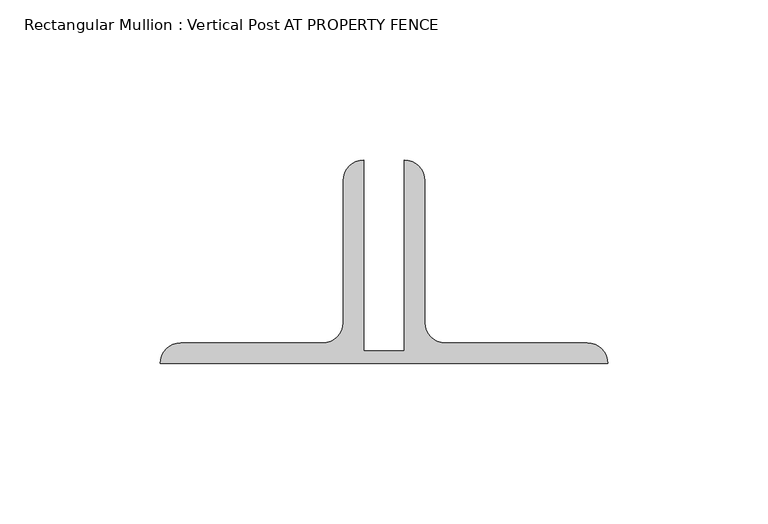
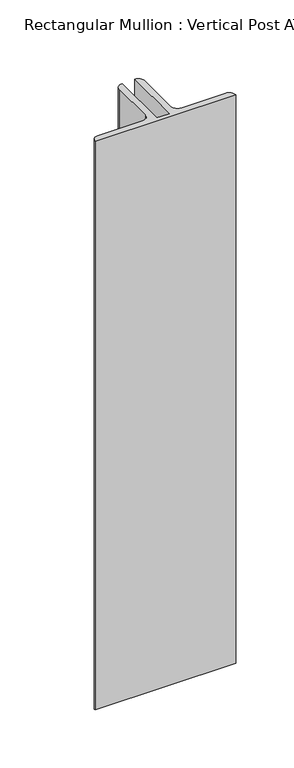
"""IFC4 building model written with IfcOpenShell, lengths in millimetres: member geometry, Rectangular Mullion : Vertical Post AT PROPERTY FENCE."""

from ifc_helpers import new_model, si_unit, point, frame, frame_2d, origin, place, context, project, spatial, polyline, circle_curve, trimmed, segment, composite_curve, outline, extrude, source, transform, mapped, element, save


def rectangular_mullion_vertical_post_at_property_fence_30249c29(model_context):
    return source(origin(), model_context, "Body", "SweptSolid", [
        extrude(outline(composite_curve([segment(polyline([(-63.5, 22.9145205), (-63.5, 82.55)]), True, "CONTINUOUS"), segment(trimmed(circle_curve(frame_2d((-63.5, 76.2)), 6.35), [point((-63.5, 82.55))], [point((-57.15, 76.2))], False, "CARTESIAN"), True, "CONTINUOUS"), segment(polyline([(-57.15, 76.2), (-57.15, 31.75)]), True, "CONTINUOUS"), segment(trimmed(circle_curve(frame_2d((-50.8, 31.75)), 6.35), [point((-57.15, 31.75))], [point((-50.8, 25.4))], True, "CARTESIAN"), True, "CONTINUOUS"), segment(polyline([(-50.8, 25.4), (-6.35, 25.4)]), True, "CONTINUOUS"), segment(trimmed(circle_curve(frame_2d((-6.35, 19.05)), 6.35), [point((-6.35, 25.4))], [point((0.0, 19.05))], False, "CARTESIAN"), True, "CONTINUOUS"), segment(polyline([(0.0, 19.05), (-139.7, 19.05)]), True, "CONTINUOUS"), segment(trimmed(circle_curve(frame_2d((-133.35, 19.05)), 6.35), [point((-139.7, 19.05))], [point((-133.35, 25.4))], False, "CARTESIAN"), True, "CONTINUOUS"), segment(polyline([(-133.35, 25.4), (-88.9, 25.4)]), True, "CONTINUOUS"), segment(trimmed(circle_curve(frame_2d((-88.9, 31.75)), 6.35), [point((-88.9, 25.4))], [point((-82.55, 31.75))], True, "CARTESIAN"), True, "CONTINUOUS"), segment(polyline([(-82.55, 31.75), (-82.55, 76.2)]), True, "CONTINUOUS"), segment(trimmed(circle_curve(frame_2d((-76.2, 76.2)), 6.35), [point((-82.55, 76.2))], [point((-76.2, 82.55))], False, "CARTESIAN"), True, "CONTINUOUS"), segment(polyline([(-76.2, 82.55), (-76.2, 22.9145205), (-63.5, 22.9145205)]), True, "CONTINUOUS")], self_intersect=False)), frame((0.0, 0.0, -596.9), z_axis=(0.0, 0.0, 1.0), x_axis=(1.0, 0.0, 0.0)), (0.0, 0.0, 1.0), 596.9),
    ])


if __name__ == "__main__":
    model = new_model("IFC4")
    model_context = context("Model", 3, world=origin())
    ifc_project = project(units=[si_unit("LENGTHUNIT", "METRE", prefix="MILLI")], contexts=[model_context])
    site = spatial("IfcSite", under=ifc_project)
    building = spatial("IfcBuilding", under=site)
    placement = place(None, origin())
    rectangular_mullion_vertical_post_at_property_fence_shape = rectangular_mullion_vertical_post_at_property_fence_30249c29(model_context)
    element("IfcMember", 1, ObjectType="Rectangular Mullion : Vertical Post AT PROPERTY FENCE", at=placement, inside=building, context=model_context, shape_type="MappedRepresentation", body=[
        mapped(rectangular_mullion_vertical_post_at_property_fence_shape, transform((0.0, 0.0, 0.0), x_axis=(1.0, 0.0, 0.0), y_axis=(0.0, 1.0, 0.0), z_axis=(0.0, 0.0, 1.0))),
    ])
    save(model, "model.ifc")

# Revit data of these elements
# Type "Rectangular Mullion : Vertical Post AT PROPERTY FENCE"
#   built-in parameter 1007351 = -0.0625 (stored number, unit not read)
#   built-in parameter 1007322 = 0.0126789 (stored number, unit not read)
#   built-in parameter 1007321 = 0.229167 (stored number, unit not read)
#   built-in parameter 1007320 = 0.229167 (stored number, unit not read)
# Element 1 (IfcMember, "Rectangular Mullion : Vertical Post AT PROPERTY FENCE")
#   Materials on its faces: "MAIN FENCE POST: (2) BACK/BACK GALVANIZED ANGLES (2) L2 1/2 X 2 1/2 X 1/4\") ANCHORED TO 8\"W X 42\" DEEP CONCRETE FOOTING(1)"
# Materials
#   "MAIN FENCE POST: (2) BACK/BACK GALVANIZED ANGLES (2) L2 1/2 X 2 1/2 X 1/4\") ANCHORED TO 8\"W X 42\" DEEP CONCRETE FOOTING(1)": class "Unassigned", colour RGB 211 211 211, transparency 0, Cost = 0
